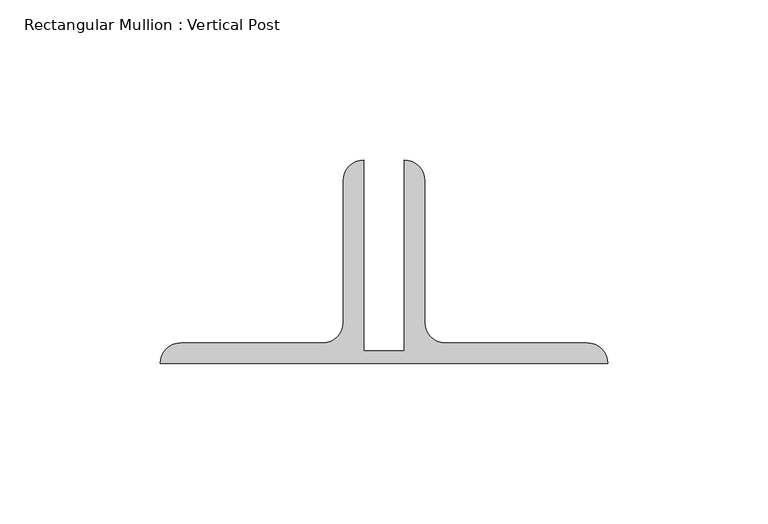
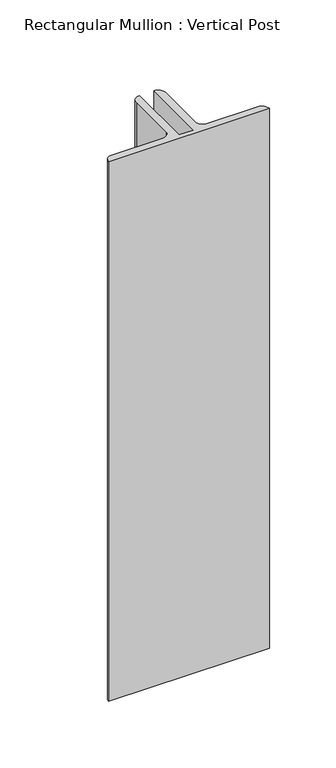
"""IFC4 building model written with IfcOpenShell, lengths in millimetres: member geometry, Rectangular Mullion : Vertical Post."""

from ifc_helpers import new_model, si_unit, point, frame, frame_2d, origin, place, context, project, spatial, polyline, circle_curve, trimmed, segment, composite_curve, outline, extrude, source, transform, mapped, element, save


def rectangular_mullion_vertical_post_c0ad3611(model_context):
    return source(origin(), model_context, "Body", "SweptSolid", [
        extrude(outline(composite_curve([segment(polyline([(-76.2, 22.9145205), (-63.5, 22.9145205), (-63.5, 82.55)]), True, "CONTINUOUS"), segment(trimmed(circle_curve(frame_2d((-63.5, 76.2)), 6.35), [point((-63.5, 82.55))], [point((-57.15, 76.2))], False, "CARTESIAN"), True, "CONTINUOUS"), segment(polyline([(-57.15, 76.2), (-57.15, 31.75)]), True, "CONTINUOUS"), segment(trimmed(circle_curve(frame_2d((-50.8, 31.75)), 6.35), [point((-57.15, 31.75))], [point((-50.8, 25.4))], True, "CARTESIAN"), True, "CONTINUOUS"), segment(polyline([(-50.8, 25.4), (-6.35, 25.4)]), True, "CONTINUOUS"), segment(trimmed(circle_curve(frame_2d((-6.35, 19.05)), 6.35), [point((-6.35, 25.4))], [point((0.0, 19.05))], False, "CARTESIAN"), True, "CONTINUOUS"), segment(polyline([(0.0, 19.05), (-139.7, 19.05)]), True, "CONTINUOUS"), segment(trimmed(circle_curve(frame_2d((-133.35, 19.05)), 6.35), [point((-139.7, 19.05))], [point((-133.35, 25.4))], False, "CARTESIAN"), True, "CONTINUOUS"), segment(polyline([(-133.35, 25.4), (-88.9, 25.4)]), True, "CONTINUOUS"), segment(trimmed(circle_curve(frame_2d((-88.9, 31.75)), 6.35), [point((-88.9, 25.4))], [point((-82.55, 31.75))], True, "CARTESIAN"), True, "CONTINUOUS"), segment(polyline([(-82.55, 31.75), (-82.55, 76.2)]), True, "CONTINUOUS"), segment(trimmed(circle_curve(frame_2d((-76.2, 76.2)), 6.35), [point((-82.55, 76.2))], [point((-76.2, 82.55))], False, "CARTESIAN"), True, "CONTINUOUS"), segment(polyline([(-76.2, 82.55), (-76.2, 22.9145205)]), True, "CONTINUOUS")], self_intersect=False)), frame((0.0, 0.0, -495.3992188), z_axis=(0.0, 0.0, 1.0), x_axis=(1.0, 0.0, 0.0)), (0.0, 0.0, 1.0), 495.3992188),
    ])


if __name__ == "__main__":
    model = new_model("IFC4")
    model_context = context("Model", 3, world=origin())
    ifc_project = project(units=[si_unit("LENGTHUNIT", "METRE", prefix="MILLI")], contexts=[model_context])
    site = spatial("IfcSite", under=ifc_project)
    building = spatial("IfcBuilding", under=site)
    placement = place(None, origin())
    rectangular_mullion_vertical_post_shape = rectangular_mullion_vertical_post_c0ad3611(model_context)
    element("IfcMember", 1, ObjectType="Rectangular Mullion : Vertical Post", at=placement, inside=building, context=model_context, shape_type="MappedRepresentation", body=[
        mapped(rectangular_mullion_vertical_post_shape, transform((0.0, 0.0, 0.0), x_axis=(1.0, 0.0, 0.0), y_axis=(0.0, 1.0, 0.0), z_axis=(0.0, 0.0, 1.0))),
    ])
    save(model, "model.ifc")

# Revit data of these elements
# Type "Rectangular Mullion : Vertical Post"
#   built-in parameter 1007351 = -0.0625 (stored number, unit not read)
#   built-in parameter 1007322 = 0.0126789 (stored number, unit not read)
#   built-in parameter 1007321 = 0.229167 (stored number, unit not read)
#   built-in parameter 1007320 = 0.229167 (stored number, unit not read)
# Element 1 (IfcMember, "Rectangular Mullion : Vertical Post")
#   Materials on its faces: "GATE POST: (2) BACK/BACK GALVANIZED ANGLES"
# Materials
#   "GATE POST: (2) BACK/BACK GALVANIZED ANGLES": class "Unassigned", colour RGB 211 211 211, transparency 0, Cost = 0
